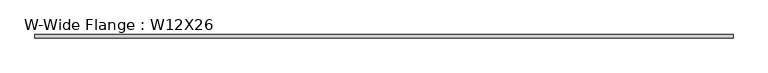
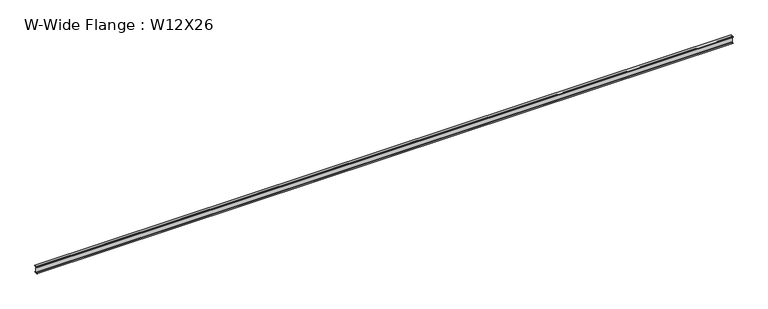
"""IFC4 building model written with IfcOpenShell, lengths in millimetres: beam geometry, W-Wide Flange : W12X26."""

import ifcopenshell
import ifcopenshell.guid

model = None  # the IFC model being written
_history = None  # IfcOwnerHistory: only IFC2X3 demands one
_inside = {}  # id of a spatial element -> (the spatial element, [elements in it])
_under = {}  # id of a project, library or spatial element -> (it, [spatial elements below it])
_declared = {}  # id of a project -> (the project, [libraries it declares])
_typed = {}  # id of a type object -> (the type object, [elements of that type])
_made_of = {}  # id of a material, layer set ... -> (it, [elements and type objects made of it])


def new_model(schema):
    """Start an empty IFC model of exactly this schema.

    Asked for "IFC4X3", IfcOpenShell would pick the latest addendum, in which some entities
    have other attributes; the version numbers below select the first issue.
    IFC2X3 requires an IfcOwnerHistory on every rooted entity: one is made here for all.
    """
    global model, _history
    if schema == "IFC4X3":
        model = ifcopenshell.file(schema_version=(4, 3, 0, 0))
    else:
        model = ifcopenshell.file(schema=schema)
    _inside.clear()
    _under.clear()
    _declared.clear()
    _typed.clear()
    _made_of.clear()
    _history = None
    if model.schema == "IFC2X3":
        org = make("IfcOrganization", Name="unknown")
        user = make(
            "IfcPersonAndOrganization",
            ThePerson=make("IfcPerson", FamilyName="unknown"),
            TheOrganization=org,
        )
        app = make(
            "IfcApplication",
            ApplicationDeveloper=org,
            Version="unknown",
            ApplicationFullName="unknown",
            ApplicationIdentifier="unknown",
        )
        _history = make(
            "IfcOwnerHistory",
            OwningUser=user,
            OwningApplication=app,
            ChangeAction="ADDED",
            CreationDate=0,
        )
    return model


def make(cls, **values):
    """One entity of the class cls with the attributes given. An attribute that is None is left unset."""
    return model.create_entity(
        cls, **{name: value for name, value in values.items() if value is not None}
    )


def rooted(cls, **values):
    """An entity with a GlobalId (a new one), such as an element, a storey or a relation."""
    return make(cls, GlobalId=ifcopenshell.guid.new(), OwnerHistory=_history, **values)


def si_unit(unit_type, name, prefix=None):
    """IfcSIUnit, for example si_unit("LENGTHUNIT", "METRE", prefix="MILLI")."""
    return make("IfcSIUnit", UnitType=unit_type, Prefix=prefix, Name=name)


def assignment(units):
    """IfcUnitAssignment: the units of a project."""
    return None if units is None else make("IfcUnitAssignment", Units=units)


def point(xyz):
    """IfcCartesianPoint."""
    return None if xyz is None else make("IfcCartesianPoint", Coordinates=xyz)


def direction(xyz):
    """IfcDirection."""
    return None if xyz is None else make("IfcDirection", DirectionRatios=xyz)


def frame(location, z_axis=None, x_axis=None):
    """IfcAxis2Placement3D, a coordinate frame: its origin and axes. An axis left out is left unset."""
    return make(
        "IfcAxis2Placement3D",
        Location=point(location),
        Axis=direction(z_axis),
        RefDirection=direction(x_axis),
    )


def frame_2d(location, x_axis=None):
    """IfcAxis2Placement2D, a coordinate frame in the plane: its origin and x axis."""
    return make(
        "IfcAxis2Placement2D", Location=point(location), RefDirection=direction(x_axis)
    )


def origin():
    """The frame at (0, 0, 0) with its axes left unset."""
    return frame((0.0, 0.0, 0.0))


def place(relative_to, where):
    """IfcLocalPlacement: puts the frame where relative to a parent placement (None: the world)."""
    return make(
        "IfcLocalPlacement", PlacementRelTo=relative_to, RelativePlacement=where
    )


def context(
    kind, dimensions, precision=None, world=None, true_north=None, identifier=None
):
    """IfcGeometricRepresentationContext, for example the 3D "Model" context."""
    return make(
        "IfcGeometricRepresentationContext",
        ContextIdentifier=identifier,
        ContextType=kind,
        CoordinateSpaceDimension=dimensions,
        Precision=precision,
        WorldCoordinateSystem=world,
        TrueNorth=true_north,
    )


def project(units=None, contexts=None):
    """IfcProject with its units and contexts."""
    return rooted(
        "IfcProject",
        Name="project",
        RepresentationContexts=contexts,
        UnitsInContext=assignment(units),
    )


def spatial(cls, under=None, at=None, **own):
    """A site, building, storey or space (cls), placed at a placement, below another one or the project."""
    s = rooted(cls, ObjectPlacement=at, **own)
    if under is not None:
        _under.setdefault(under.id(), (under, []))[1].append(s)
    return s


def polyline(points):
    """IfcPolyline through the points."""
    return make("IfcPolyline", Points=[point(p) for p in points])


def circle_curve(where, radius):
    """IfcCircle in the frame where."""
    return make("IfcCircle", Position=where, Radius=radius)


def trimmed(basis, trim1, trim2, sense, master):
    """IfcTrimmedCurve: the piece of a basis curve between two trims."""
    return make(
        "IfcTrimmedCurve",
        BasisCurve=basis,
        Trim1=trim1,
        Trim2=trim2,
        SenseAgreement=sense,
        MasterRepresentation=master,
    )


def segment(curve, same_sense, transition):
    """IfcCompositeCurveSegment."""
    return make(
        "IfcCompositeCurveSegment",
        Transition=transition,
        SameSense=same_sense,
        ParentCurve=curve,
    )


def composite_curve(segments, self_intersect=None):
    """IfcCompositeCurve: segments joined end to end."""
    return make("IfcCompositeCurve", Segments=segments, SelfIntersect=self_intersect)


def outline(outer, holes=None, kind="AREA"):
    """IfcArbitraryClosedProfileDef: a profile drawn as a closed curve; with holes, ...WithVoids."""
    if holes is None:
        return make("IfcArbitraryClosedProfileDef", ProfileType=kind, OuterCurve=outer)
    return make(
        "IfcArbitraryProfileDefWithVoids",
        ProfileType=kind,
        OuterCurve=outer,
        InnerCurves=holes,
    )


def extrude(swept, where, along, depth):
    """IfcExtrudedAreaSolid: the profile swept, set in the frame where, extruded along a direction by depth."""
    return make(
        "IfcExtrudedAreaSolid",
        SweptArea=swept,
        Position=where,
        ExtrudedDirection=direction(along),
        Depth=depth,
    )


def shape(context_of_items, identifier, shape_type, items):
    """IfcShapeRepresentation: the items that make up one representation, for example the "Body"."""
    return make(
        "IfcShapeRepresentation",
        ContextOfItems=context_of_items,
        RepresentationIdentifier=identifier,
        RepresentationType=shape_type,
        Items=items,
    )


def source(mapping_origin, context_of_items, identifier, shape_type, items):
    """IfcRepresentationMap: a shape defined once, which mapped items show again and again."""
    return make(
        "IfcRepresentationMap",
        MappingOrigin=mapping_origin,
        MappedRepresentation=shape(context_of_items, identifier, shape_type, items),
    )


def transform(
    local_origin,
    x_axis=None,
    y_axis=None,
    z_axis=None,
    scale=None,
    scale2=None,
    scale3=None,
    uniform=True,
):
    """IfcCartesianTransformationOperator3D, or its non-uniform kind. x_axis, y_axis, z_axis: its Axis1, 2, 3."""
    if uniform:
        return make(
            "IfcCartesianTransformationOperator3D",
            Axis1=direction(x_axis),
            Axis2=direction(y_axis),
            LocalOrigin=point(local_origin),
            Scale=scale,
            Axis3=direction(z_axis),
        )
    return make(
        "IfcCartesianTransformationOperator3DnonUniform",
        Axis1=direction(x_axis),
        Axis2=direction(y_axis),
        LocalOrigin=point(local_origin),
        Scale=scale,
        Axis3=direction(z_axis),
        Scale2=scale2,
        Scale3=scale3,
    )


def mapped(mapping_source, mapping_target):
    """IfcMappedItem: shows the shape of a source again, moved by a transform."""
    return make(
        "IfcMappedItem", MappingSource=mapping_source, MappingTarget=mapping_target
    )


def made_of(thing, what):
    """Note that an element or type object is made of a material, layer set ...; save() writes the relation."""
    if what is not None:
        _made_of.setdefault(what.id(), (what, []))[1].append(thing)
    return thing


def element(
    cls,
    number,
    at=None,
    inside=None,
    cuts=None,
    type_object=None,
    material=None,
    context=None,
    identifier="Body",
    shape_type=None,
    held_by="IfcProductDefinitionShape",
    body=None,
    shapes=None,
    **own,
):
    """One element of the class cls, such as IfcWall. Its Tag is "e" and its number.

    at: its placement. inside: the storey or other place that contains it. cuts: it is an
    opening in that element (IfcRelVoidsElement). A single representation is given by context,
    identifier, shape_type and body (its items); several are given by shapes. held_by: the class
    of the entity that holds the representations. save() writes the other relations.
    """
    e = rooted(cls, Tag="e%d" % number, ObjectPlacement=at, **own)
    if body is not None:
        shapes = [shape(context, identifier, shape_type, body)]
    if shapes is not None:
        e.Representation = make(held_by, Representations=shapes)
    if inside is not None:
        _inside.setdefault(inside.id(), (inside, []))[1].append(e)
    if cuts is not None:
        rooted(
            "IfcRelVoidsElement", RelatingBuildingElement=cuts, RelatedOpeningElement=e
        )
    if type_object is not None:
        _typed.setdefault(type_object.id(), (type_object, []))[1].append(e)
    return made_of(e, material)


def aggregate(whole, parts):
    """IfcRelAggregates: a whole, such as a stair, and the parts it consists of."""
    return rooted("IfcRelAggregates", RelatingObject=whole, RelatedObjects=parts)


def save(model, path):
    """Write the relations noted so far, then the file.

    IfcRelAggregates (storeys below a building ...), IfcRelContainedInSpatialStructure (elements
    in a storey), IfcRelDefinesByType, IfcRelAssociatesMaterial and IfcRelDeclares: one each for
    every whole, place, type object, material and project.
    """
    for whole, parts in _under.values():
        aggregate(whole, parts)
    for where, things in _inside.values():
        rooted(
            "IfcRelContainedInSpatialStructure",
            RelatedElements=things,
            RelatingStructure=where,
        )
    for kind, things in _typed.values():
        rooted("IfcRelDefinesByType", RelatedObjects=things, RelatingType=kind)
    for what, things in _made_of.values():
        rooted("IfcRelAssociatesMaterial", RelatedObjects=things, RelatingMaterial=what)
    for by, libraries in _declared.values():
        rooted("IfcRelDeclares", RelatingContext=by, RelatedDefinitions=libraries)
    model.write(path)


def w_wide_flange_w12x26_a5ed678c(model_context):
    return source(origin(), model_context, "Body", "SweptSolid", [
        extrude(outline(composite_curve([segment(polyline([(82.4011719, -145.5539063), (82.4011719, -155.178125), (-82.4011719, -155.178125), (-82.4011719, -145.5539063), (-20.2902344, -145.5539063)]), True, "CONTINUOUS"), segment(trimmed(circle_curve(frame_2d((-20.2902344, -128.190625)), 17.3632812), [point((-20.2902344, -145.5539063))], [point((-2.9269531, -128.190625))], True, "CARTESIAN"), True, "CONTINUOUS"), segment(polyline([(-2.9269531, -128.190625), (-2.9269531, 128.190625)]), True, "CONTINUOUS"), segment(trimmed(circle_curve(frame_2d((-20.2902344, 128.190625)), 17.3632812), [point((-2.9269531, 128.190625))], [point((-20.2902344, 145.5539062))], True, "CARTESIAN"), True, "CONTINUOUS"), segment(polyline([(-20.2902344, 145.5539062), (-82.4011719, 145.5539062), (-82.4011719, 155.178125), (82.4011719, 155.178125), (82.4011719, 145.5539062), (20.2902344, 145.5539062)]), True, "CONTINUOUS"), segment(trimmed(circle_curve(frame_2d((20.2902344, 128.190625)), 17.3632812), [point((20.2902344, 145.5539062))], [point((2.9269531, 128.190625))], True, "CARTESIAN"), True, "CONTINUOUS"), segment(polyline([(2.9269531, 128.190625), (2.9269531, -128.190625)]), True, "CONTINUOUS"), segment(trimmed(circle_curve(frame_2d((20.2902344, -128.190625)), 17.3632812), [point((2.9269531, -128.190625))], [point((20.2902344, -145.5539063))], True, "CARTESIAN"), True, "CONTINUOUS"), segment(polyline([(20.2902344, -145.5539063), (82.4011719, -145.5539063)]), True, "CONTINUOUS")], self_intersect=False)), frame((-16262.75233, 0.0, 0.0), z_axis=(1.0, 0.0, 0.0), x_axis=(0.0, 1.0, 0.0)), (0.0, 0.0, 1.0), 32561.1761131),
    ])


if __name__ == "__main__":
    model = new_model("IFC4")
    model_context = context("Model", 3, world=origin())
    ifc_project = project(units=[si_unit("LENGTHUNIT", "METRE", prefix="MILLI")], contexts=[model_context])
    site = spatial("IfcSite", under=ifc_project)
    building = spatial("IfcBuilding", under=site)
    placement = place(None, origin())
    w_wide_flange_w12x26_shape = w_wide_flange_w12x26_a5ed678c(model_context)
    element("IfcBeam", 1, ObjectType="W-Wide Flange : W12X26", at=placement, inside=building, context=model_context, shape_type="MappedRepresentation", body=[
        mapped(w_wide_flange_w12x26_shape, transform((0.0, 0.0, 0.0), x_axis=(1.0, 0.0, 0.0), y_axis=(0.0, 1.0, 0.0), z_axis=(0.0, 0.0, 1.0))),
    ])
    save(model, "model.ifc")

# Revit data of these elements
# Type "W-Wide Flange : W12X26"
#   Assembly Code = "B10"
#   W = 26
#   Length [instance default] = 5' - 0"
#   bf = 0' - 6 125/256"
#   d = 1' - 0 7/32"
#   k = 0' - 1 1/16"
#   k2 = 0' - 0 175/256"
#   tf = 0' - 0 97/256"
#   tw = 0' - 0 59/256"
#   A = 0.053125 SF
#   Structural Material [instance default] = none
